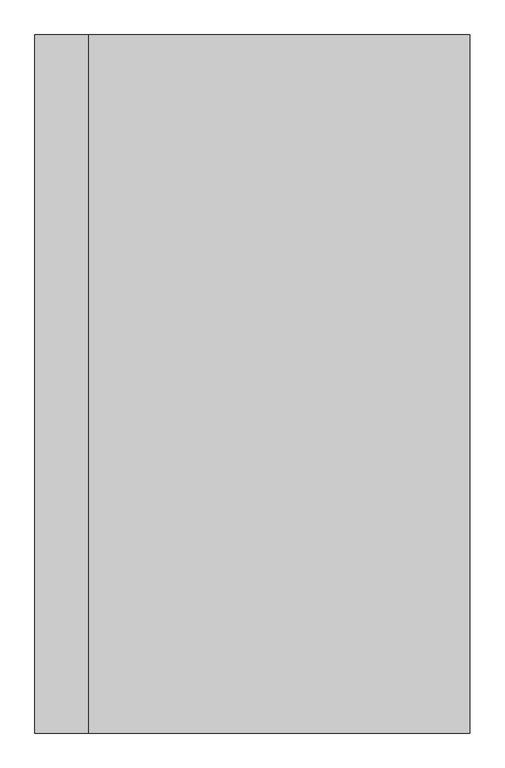
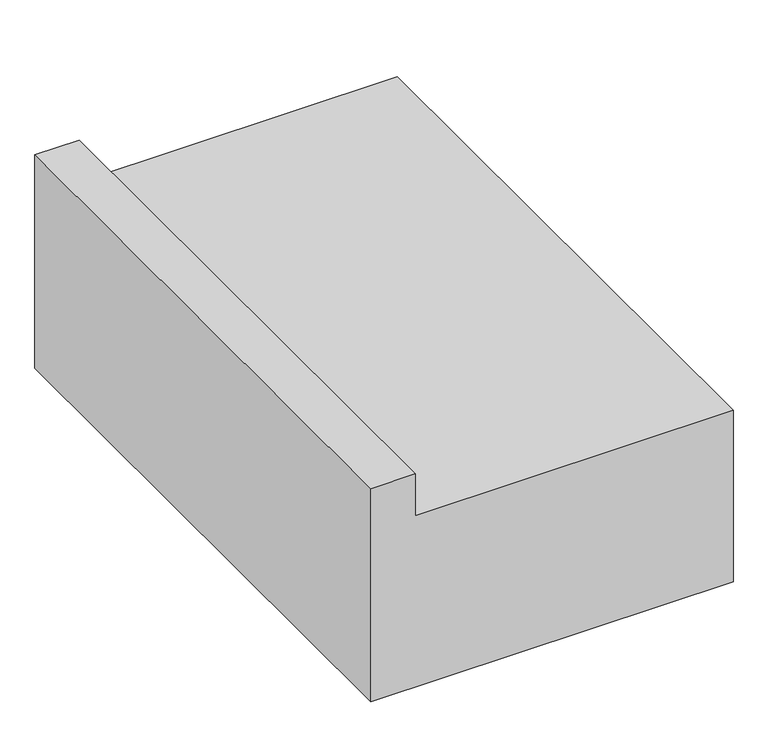
"""IFC4 building model written with IfcOpenShell, lengths in millimetres: proxy geometry, Structure069 6054 : Structure069 6054."""

import ifcopenshell
import ifcopenshell.guid

model = None  # the IFC model being written
_history = None  # IfcOwnerHistory: only IFC2X3 demands one
_inside = {}  # id of a spatial element -> (the spatial element, [elements in it])
_under = {}  # id of a project, library or spatial element -> (it, [spatial elements below it])
_declared = {}  # id of a project -> (the project, [libraries it declares])
_typed = {}  # id of a type object -> (the type object, [elements of that type])
_made_of = {}  # id of a material, layer set ... -> (it, [elements and type objects made of it])


def new_model(schema):
    """Start an empty IFC model of exactly this schema.

    Asked for "IFC4X3", IfcOpenShell would pick the latest addendum, in which some entities
    have other attributes; the version numbers below select the first issue.
    IFC2X3 requires an IfcOwnerHistory on every rooted entity: one is made here for all.
    """
    global model, _history
    if schema == "IFC4X3":
        model = ifcopenshell.file(schema_version=(4, 3, 0, 0))
    else:
        model = ifcopenshell.file(schema=schema)
    _inside.clear()
    _under.clear()
    _declared.clear()
    _typed.clear()
    _made_of.clear()
    _history = None
    if model.schema == "IFC2X3":
        org = make("IfcOrganization", Name="unknown")
        user = make(
            "IfcPersonAndOrganization",
            ThePerson=make("IfcPerson", FamilyName="unknown"),
            TheOrganization=org,
        )
        app = make(
            "IfcApplication",
            ApplicationDeveloper=org,
            Version="unknown",
            ApplicationFullName="unknown",
            ApplicationIdentifier="unknown",
        )
        _history = make(
            "IfcOwnerHistory",
            OwningUser=user,
            OwningApplication=app,
            ChangeAction="ADDED",
            CreationDate=0,
        )
    return model


def make(cls, **values):
    """One entity of the class cls with the attributes given. An attribute that is None is left unset."""
    return model.create_entity(
        cls, **{name: value for name, value in values.items() if value is not None}
    )


def rooted(cls, **values):
    """An entity with a GlobalId (a new one), such as an element, a storey or a relation."""
    return make(cls, GlobalId=ifcopenshell.guid.new(), OwnerHistory=_history, **values)


def si_unit(unit_type, name, prefix=None):
    """IfcSIUnit, for example si_unit("LENGTHUNIT", "METRE", prefix="MILLI")."""
    return make("IfcSIUnit", UnitType=unit_type, Prefix=prefix, Name=name)


def assignment(units):
    """IfcUnitAssignment: the units of a project."""
    return None if units is None else make("IfcUnitAssignment", Units=units)


def point(xyz):
    """IfcCartesianPoint."""
    return None if xyz is None else make("IfcCartesianPoint", Coordinates=xyz)


def direction(xyz):
    """IfcDirection."""
    return None if xyz is None else make("IfcDirection", DirectionRatios=xyz)


def frame(location, z_axis=None, x_axis=None):
    """IfcAxis2Placement3D, a coordinate frame: its origin and axes. An axis left out is left unset."""
    return make(
        "IfcAxis2Placement3D",
        Location=point(location),
        Axis=direction(z_axis),
        RefDirection=direction(x_axis),
    )


def origin():
    """The frame at (0, 0, 0) with its axes left unset."""
    return frame((0.0, 0.0, 0.0))


def place(relative_to, where):
    """IfcLocalPlacement: puts the frame where relative to a parent placement (None: the world)."""
    return make(
        "IfcLocalPlacement", PlacementRelTo=relative_to, RelativePlacement=where
    )


def context(
    kind, dimensions, precision=None, world=None, true_north=None, identifier=None
):
    """IfcGeometricRepresentationContext, for example the 3D "Model" context."""
    return make(
        "IfcGeometricRepresentationContext",
        ContextIdentifier=identifier,
        ContextType=kind,
        CoordinateSpaceDimension=dimensions,
        Precision=precision,
        WorldCoordinateSystem=world,
        TrueNorth=true_north,
    )


def project(units=None, contexts=None):
    """IfcProject with its units and contexts."""
    return rooted(
        "IfcProject",
        Name="project",
        RepresentationContexts=contexts,
        UnitsInContext=assignment(units),
    )


def spatial(cls, under=None, at=None, **own):
    """A site, building, storey or space (cls), placed at a placement, below another one or the project."""
    s = rooted(cls, ObjectPlacement=at, **own)
    if under is not None:
        _under.setdefault(under.id(), (under, []))[1].append(s)
    return s


def polyline(points):
    """IfcPolyline through the points."""
    return make("IfcPolyline", Points=[point(p) for p in points])


def outline(outer, holes=None, kind="AREA"):
    """IfcArbitraryClosedProfileDef: a profile drawn as a closed curve; with holes, ...WithVoids."""
    if holes is None:
        return make("IfcArbitraryClosedProfileDef", ProfileType=kind, OuterCurve=outer)
    return make(
        "IfcArbitraryProfileDefWithVoids",
        ProfileType=kind,
        OuterCurve=outer,
        InnerCurves=holes,
    )


def extrude(swept, where, along, depth):
    """IfcExtrudedAreaSolid: the profile swept, set in the frame where, extruded along a direction by depth."""
    return make(
        "IfcExtrudedAreaSolid",
        SweptArea=swept,
        Position=where,
        ExtrudedDirection=direction(along),
        Depth=depth,
    )


def shape(context_of_items, identifier, shape_type, items):
    """IfcShapeRepresentation: the items that make up one representation, for example the "Body"."""
    return make(
        "IfcShapeRepresentation",
        ContextOfItems=context_of_items,
        RepresentationIdentifier=identifier,
        RepresentationType=shape_type,
        Items=items,
    )


def source(mapping_origin, context_of_items, identifier, shape_type, items):
    """IfcRepresentationMap: a shape defined once, which mapped items show again and again."""
    return make(
        "IfcRepresentationMap",
        MappingOrigin=mapping_origin,
        MappedRepresentation=shape(context_of_items, identifier, shape_type, items),
    )


def transform(
    local_origin,
    x_axis=None,
    y_axis=None,
    z_axis=None,
    scale=None,
    scale2=None,
    scale3=None,
    uniform=True,
):
    """IfcCartesianTransformationOperator3D, or its non-uniform kind. x_axis, y_axis, z_axis: its Axis1, 2, 3."""
    if uniform:
        return make(
            "IfcCartesianTransformationOperator3D",
            Axis1=direction(x_axis),
            Axis2=direction(y_axis),
            LocalOrigin=point(local_origin),
            Scale=scale,
            Axis3=direction(z_axis),
        )
    return make(
        "IfcCartesianTransformationOperator3DnonUniform",
        Axis1=direction(x_axis),
        Axis2=direction(y_axis),
        LocalOrigin=point(local_origin),
        Scale=scale,
        Axis3=direction(z_axis),
        Scale2=scale2,
        Scale3=scale3,
    )


def mapped(mapping_source, mapping_target):
    """IfcMappedItem: shows the shape of a source again, moved by a transform."""
    return make(
        "IfcMappedItem", MappingSource=mapping_source, MappingTarget=mapping_target
    )


def made_of(thing, what):
    """Note that an element or type object is made of a material, layer set ...; save() writes the relation."""
    if what is not None:
        _made_of.setdefault(what.id(), (what, []))[1].append(thing)
    return thing


def element(
    cls,
    number,
    at=None,
    inside=None,
    cuts=None,
    type_object=None,
    material=None,
    context=None,
    identifier="Body",
    shape_type=None,
    held_by="IfcProductDefinitionShape",
    body=None,
    shapes=None,
    **own,
):
    """One element of the class cls, such as IfcWall. Its Tag is "e" and its number.

    at: its placement. inside: the storey or other place that contains it. cuts: it is an
    opening in that element (IfcRelVoidsElement). A single representation is given by context,
    identifier, shape_type and body (its items); several are given by shapes. held_by: the class
    of the entity that holds the representations. save() writes the other relations.
    """
    e = rooted(cls, Tag="e%d" % number, ObjectPlacement=at, **own)
    if body is not None:
        shapes = [shape(context, identifier, shape_type, body)]
    if shapes is not None:
        e.Representation = make(held_by, Representations=shapes)
    if inside is not None:
        _inside.setdefault(inside.id(), (inside, []))[1].append(e)
    if cuts is not None:
        rooted(
            "IfcRelVoidsElement", RelatingBuildingElement=cuts, RelatedOpeningElement=e
        )
    if type_object is not None:
        _typed.setdefault(type_object.id(), (type_object, []))[1].append(e)
    return made_of(e, material)


def aggregate(whole, parts):
    """IfcRelAggregates: a whole, such as a stair, and the parts it consists of."""
    return rooted("IfcRelAggregates", RelatingObject=whole, RelatedObjects=parts)


def save(model, path):
    """Write the relations noted so far, then the file.

    IfcRelAggregates (storeys below a building ...), IfcRelContainedInSpatialStructure (elements
    in a storey), IfcRelDefinesByType, IfcRelAssociatesMaterial and IfcRelDeclares: one each for
    every whole, place, type object, material and project.
    """
    for whole, parts in _under.values():
        aggregate(whole, parts)
    for where, things in _inside.values():
        rooted(
            "IfcRelContainedInSpatialStructure",
            RelatedElements=things,
            RelatingStructure=where,
        )
    for kind, things in _typed.values():
        rooted("IfcRelDefinesByType", RelatedObjects=things, RelatingType=kind)
    for what, things in _made_of.values():
        rooted("IfcRelAssociatesMaterial", RelatedObjects=things, RelatingMaterial=what)
    for by, libraries in _declared.values():
        rooted("IfcRelDeclares", RelatingContext=by, RelatedDefinitions=libraries)
    model.write(path)


def generic_models_5d2a26bb(model_context):
    return source(origin(), model_context, "Body", "SweptSolid", [
        extrude(outline(polyline([(36112.196, 11291.2000945), (36734.496, 11291.2000945), (36734.496, 10197.8052734), (36886.896, 10197.8052734), (36886.896, 10045.4052734), (36112.196, 10045.4052734), (36112.196, 11291.2000945)])), frame((0.0, 2217.3609988, 0.0), z_axis=(0.0, 1.0, 0.0), x_axis=(0.0, 0.0, 1.0)), (0.0, 0.0, 1.0), 2000.0),
    ])


if __name__ == "__main__":
    model = new_model("IFC4")
    model_context = context("Model", 3, world=origin())
    ifc_project = project(units=[si_unit("LENGTHUNIT", "METRE", prefix="MILLI")], contexts=[model_context])
    site = spatial("IfcSite", under=ifc_project)
    building = spatial("IfcBuilding", under=site)
    placement = place(None, origin())
    generic_models_shape = generic_models_5d2a26bb(model_context)
    element("IfcBuildingElementProxy", 1, Name="Structure069 6054 : Structure069 6054", ObjectType="Structure069 6054 : Structure069 6054", at=placement, inside=building, context=model_context, shape_type="MappedRepresentation", body=[
        mapped(generic_models_shape, transform((0.0, 0.0, 0.0), x_axis=(1.0, 0.0, 0.0), y_axis=(0.0, 1.0, 0.0), z_axis=(0.0, 0.0, 1.0))),
    ])
    save(model, "model.ifc")

# Revit data of these elements
# Type "Structure069 6054 : Structure069 6054"
#   NameOverride = "Structure069"
# Element 1 (IfcBuildingElementProxy, "Structure069 6054 : Structure069 6054")
#   Materials on its faces: "CONCRETE SLAB W/ GRADE BEAM (SEE STRUCT DWGS)"
# Materials
#   "CONCRETE SLAB W/ GRADE BEAM (SEE STRUCT DWGS)": class "Unassigned", colour RGB 128 128 128, transparency 0, Cost = 0
